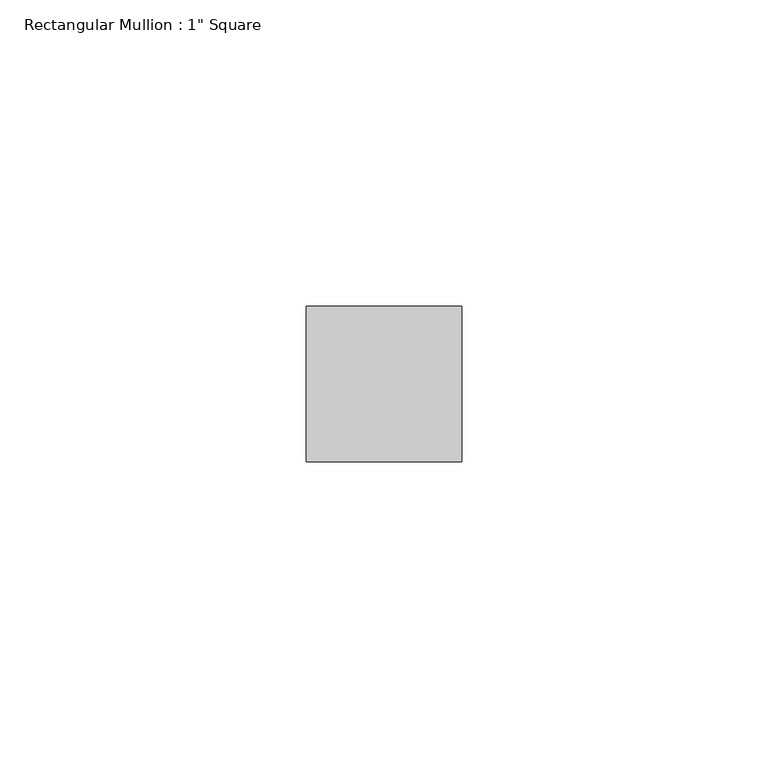
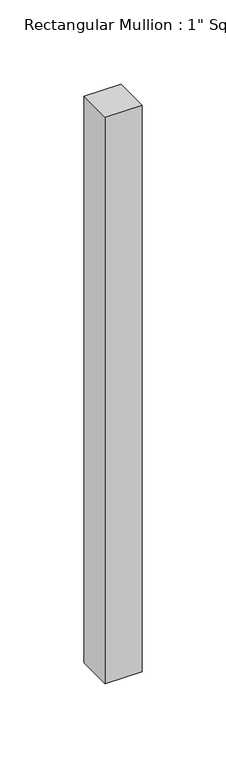
"""IFC4 building model written with IfcOpenShell, lengths in millimetres: member geometry."""

from ifc_helpers import new_model, si_unit, frame, origin, place, context, project, spatial, polyline, outline, extrude, source, transform, mapped, element, save


def member_9fdc781f(model_context):
    return source(origin(), model_context, "Body", "SweptSolid", [
        extrude(outline(polyline([(12.7, 12.7), (12.7, -12.7), (-12.7, -12.7), (-12.7, 12.7), (12.7, 12.7)])), frame((0.0, 0.0, -411.4022832), z_axis=(0.0, 0.0, 1.0), x_axis=(1.0, 0.0, 0.0)), (0.0, 0.0, 1.0), 411.4022832),
    ])


if __name__ == "__main__":
    model = new_model("IFC4")
    model_context = context("Model", 3, world=origin())
    ifc_project = project(units=[si_unit("LENGTHUNIT", "METRE", prefix="MILLI")], contexts=[model_context])
    site = spatial("IfcSite", under=ifc_project)
    building = spatial("IfcBuilding", under=site)
    placement = place(None, origin())
    member_shape = member_9fdc781f(model_context)
    element("IfcMember", 1, ObjectType="Rectangular Mullion : 1\" Square", at=placement, inside=building, context=model_context, shape_type="MappedRepresentation", body=[
        mapped(member_shape, transform((0.0, 0.0, 0.0), x_axis=(1.0, 0.0, 0.0), y_axis=(0.0, 1.0, 0.0), z_axis=(0.0, 0.0, 1.0))),
    ])
    save(model, "model.ifc")

# Revit data of these elements
# Type "Rectangular Mullion : 1\" Square"
#   built-in parameter 1007304 = 0.0833333 (stored number, unit not read)
#   built-in parameter 1007301 = 0.0416667 (stored number, unit not read)
#   built-in parameter 1007300 = 0.0416667 (stored number, unit not read)
# Element 1 (IfcMember, "Rectangular Mullion : 1\" Square")
#   Materials on its faces: "Metal - Aluminum"
# Materials
#   "Metal - Aluminum": class "Metal", colour RGB 247 247 247, transparency 0
